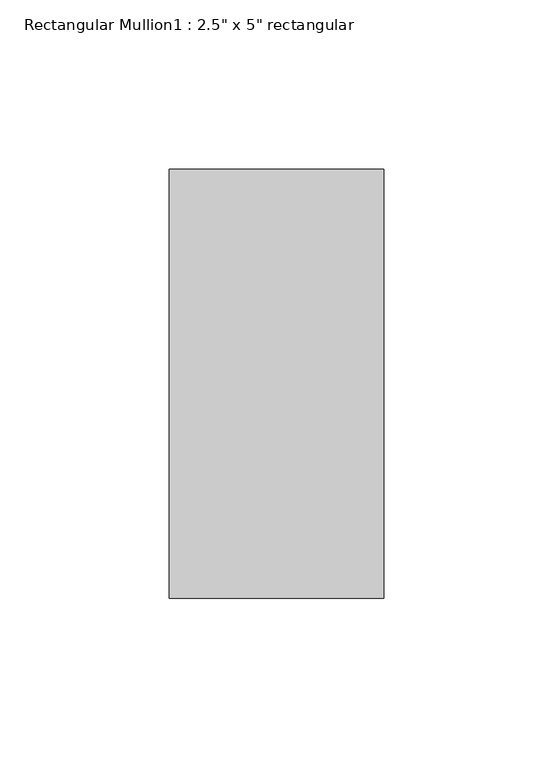
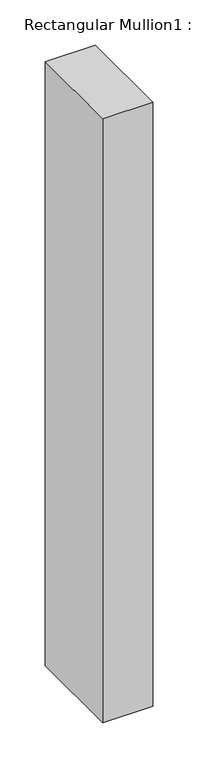
"""IFC4 building model written with IfcOpenShell, lengths in millimetres: member geometry."""

import ifcopenshell
import ifcopenshell.guid

model = None  # the IFC model being written
_history = None  # IfcOwnerHistory: only IFC2X3 demands one
_inside = {}  # id of a spatial element -> (the spatial element, [elements in it])
_under = {}  # id of a project, library or spatial element -> (it, [spatial elements below it])
_declared = {}  # id of a project -> (the project, [libraries it declares])
_typed = {}  # id of a type object -> (the type object, [elements of that type])
_made_of = {}  # id of a material, layer set ... -> (it, [elements and type objects made of it])


def new_model(schema):
    """Start an empty IFC model of exactly this schema.

    Asked for "IFC4X3", IfcOpenShell would pick the latest addendum, in which some entities
    have other attributes; the version numbers below select the first issue.
    IFC2X3 requires an IfcOwnerHistory on every rooted entity: one is made here for all.
    """
    global model, _history
    if schema == "IFC4X3":
        model = ifcopenshell.file(schema_version=(4, 3, 0, 0))
    else:
        model = ifcopenshell.file(schema=schema)
    _inside.clear()
    _under.clear()
    _declared.clear()
    _typed.clear()
    _made_of.clear()
    _history = None
    if model.schema == "IFC2X3":
        org = make("IfcOrganization", Name="unknown")
        user = make(
            "IfcPersonAndOrganization",
            ThePerson=make("IfcPerson", FamilyName="unknown"),
            TheOrganization=org,
        )
        app = make(
            "IfcApplication",
            ApplicationDeveloper=org,
            Version="unknown",
            ApplicationFullName="unknown",
            ApplicationIdentifier="unknown",
        )
        _history = make(
            "IfcOwnerHistory",
            OwningUser=user,
            OwningApplication=app,
            ChangeAction="ADDED",
            CreationDate=0,
        )
    return model


def make(cls, **values):
    """One entity of the class cls with the attributes given. An attribute that is None is left unset."""
    return model.create_entity(
        cls, **{name: value for name, value in values.items() if value is not None}
    )


def rooted(cls, **values):
    """An entity with a GlobalId (a new one), such as an element, a storey or a relation."""
    return make(cls, GlobalId=ifcopenshell.guid.new(), OwnerHistory=_history, **values)


def si_unit(unit_type, name, prefix=None):
    """IfcSIUnit, for example si_unit("LENGTHUNIT", "METRE", prefix="MILLI")."""
    return make("IfcSIUnit", UnitType=unit_type, Prefix=prefix, Name=name)


def assignment(units):
    """IfcUnitAssignment: the units of a project."""
    return None if units is None else make("IfcUnitAssignment", Units=units)


def point(xyz):
    """IfcCartesianPoint."""
    return None if xyz is None else make("IfcCartesianPoint", Coordinates=xyz)


def direction(xyz):
    """IfcDirection."""
    return None if xyz is None else make("IfcDirection", DirectionRatios=xyz)


def frame(location, z_axis=None, x_axis=None):
    """IfcAxis2Placement3D, a coordinate frame: its origin and axes. An axis left out is left unset."""
    return make(
        "IfcAxis2Placement3D",
        Location=point(location),
        Axis=direction(z_axis),
        RefDirection=direction(x_axis),
    )


def origin():
    """The frame at (0, 0, 0) with its axes left unset."""
    return frame((0.0, 0.0, 0.0))


def place(relative_to, where):
    """IfcLocalPlacement: puts the frame where relative to a parent placement (None: the world)."""
    return make(
        "IfcLocalPlacement", PlacementRelTo=relative_to, RelativePlacement=where
    )


def context(
    kind, dimensions, precision=None, world=None, true_north=None, identifier=None
):
    """IfcGeometricRepresentationContext, for example the 3D "Model" context."""
    return make(
        "IfcGeometricRepresentationContext",
        ContextIdentifier=identifier,
        ContextType=kind,
        CoordinateSpaceDimension=dimensions,
        Precision=precision,
        WorldCoordinateSystem=world,
        TrueNorth=true_north,
    )


def project(units=None, contexts=None):
    """IfcProject with its units and contexts."""
    return rooted(
        "IfcProject",
        Name="project",
        RepresentationContexts=contexts,
        UnitsInContext=assignment(units),
    )


def spatial(cls, under=None, at=None, **own):
    """A site, building, storey or space (cls), placed at a placement, below another one or the project."""
    s = rooted(cls, ObjectPlacement=at, **own)
    if under is not None:
        _under.setdefault(under.id(), (under, []))[1].append(s)
    return s


def polyline(points):
    """IfcPolyline through the points."""
    return make("IfcPolyline", Points=[point(p) for p in points])


def outline(outer, holes=None, kind="AREA"):
    """IfcArbitraryClosedProfileDef: a profile drawn as a closed curve; with holes, ...WithVoids."""
    if holes is None:
        return make("IfcArbitraryClosedProfileDef", ProfileType=kind, OuterCurve=outer)
    return make(
        "IfcArbitraryProfileDefWithVoids",
        ProfileType=kind,
        OuterCurve=outer,
        InnerCurves=holes,
    )


def extrude(swept, where, along, depth):
    """IfcExtrudedAreaSolid: the profile swept, set in the frame where, extruded along a direction by depth."""
    return make(
        "IfcExtrudedAreaSolid",
        SweptArea=swept,
        Position=where,
        ExtrudedDirection=direction(along),
        Depth=depth,
    )


def shape(context_of_items, identifier, shape_type, items):
    """IfcShapeRepresentation: the items that make up one representation, for example the "Body"."""
    return make(
        "IfcShapeRepresentation",
        ContextOfItems=context_of_items,
        RepresentationIdentifier=identifier,
        RepresentationType=shape_type,
        Items=items,
    )


def source(mapping_origin, context_of_items, identifier, shape_type, items):
    """IfcRepresentationMap: a shape defined once, which mapped items show again and again."""
    return make(
        "IfcRepresentationMap",
        MappingOrigin=mapping_origin,
        MappedRepresentation=shape(context_of_items, identifier, shape_type, items),
    )


def transform(
    local_origin,
    x_axis=None,
    y_axis=None,
    z_axis=None,
    scale=None,
    scale2=None,
    scale3=None,
    uniform=True,
):
    """IfcCartesianTransformationOperator3D, or its non-uniform kind. x_axis, y_axis, z_axis: its Axis1, 2, 3."""
    if uniform:
        return make(
            "IfcCartesianTransformationOperator3D",
            Axis1=direction(x_axis),
            Axis2=direction(y_axis),
            LocalOrigin=point(local_origin),
            Scale=scale,
            Axis3=direction(z_axis),
        )
    return make(
        "IfcCartesianTransformationOperator3DnonUniform",
        Axis1=direction(x_axis),
        Axis2=direction(y_axis),
        LocalOrigin=point(local_origin),
        Scale=scale,
        Axis3=direction(z_axis),
        Scale2=scale2,
        Scale3=scale3,
    )


def mapped(mapping_source, mapping_target):
    """IfcMappedItem: shows the shape of a source again, moved by a transform."""
    return make(
        "IfcMappedItem", MappingSource=mapping_source, MappingTarget=mapping_target
    )


def made_of(thing, what):
    """Note that an element or type object is made of a material, layer set ...; save() writes the relation."""
    if what is not None:
        _made_of.setdefault(what.id(), (what, []))[1].append(thing)
    return thing


def element(
    cls,
    number,
    at=None,
    inside=None,
    cuts=None,
    type_object=None,
    material=None,
    context=None,
    identifier="Body",
    shape_type=None,
    held_by="IfcProductDefinitionShape",
    body=None,
    shapes=None,
    **own,
):
    """One element of the class cls, such as IfcWall. Its Tag is "e" and its number.

    at: its placement. inside: the storey or other place that contains it. cuts: it is an
    opening in that element (IfcRelVoidsElement). A single representation is given by context,
    identifier, shape_type and body (its items); several are given by shapes. held_by: the class
    of the entity that holds the representations. save() writes the other relations.
    """
    e = rooted(cls, Tag="e%d" % number, ObjectPlacement=at, **own)
    if body is not None:
        shapes = [shape(context, identifier, shape_type, body)]
    if shapes is not None:
        e.Representation = make(held_by, Representations=shapes)
    if inside is not None:
        _inside.setdefault(inside.id(), (inside, []))[1].append(e)
    if cuts is not None:
        rooted(
            "IfcRelVoidsElement", RelatingBuildingElement=cuts, RelatedOpeningElement=e
        )
    if type_object is not None:
        _typed.setdefault(type_object.id(), (type_object, []))[1].append(e)
    return made_of(e, material)


def aggregate(whole, parts):
    """IfcRelAggregates: a whole, such as a stair, and the parts it consists of."""
    return rooted("IfcRelAggregates", RelatingObject=whole, RelatedObjects=parts)


def save(model, path):
    """Write the relations noted so far, then the file.

    IfcRelAggregates (storeys below a building ...), IfcRelContainedInSpatialStructure (elements
    in a storey), IfcRelDefinesByType, IfcRelAssociatesMaterial and IfcRelDeclares: one each for
    every whole, place, type object, material and project.
    """
    for whole, parts in _under.values():
        aggregate(whole, parts)
    for where, things in _inside.values():
        rooted(
            "IfcRelContainedInSpatialStructure",
            RelatedElements=things,
            RelatingStructure=where,
        )
    for kind, things in _typed.values():
        rooted("IfcRelDefinesByType", RelatedObjects=things, RelatingType=kind)
    for what, things in _made_of.values():
        rooted("IfcRelAssociatesMaterial", RelatedObjects=things, RelatingMaterial=what)
    for by, libraries in _declared.values():
        rooted("IfcRelDeclares", RelatingContext=by, RelatedDefinitions=libraries)
    model.write(path)


def member_7227ddca(model_context):
    return source(origin(), model_context, "Body", "SweptSolid", [
        extrude(outline(polyline([(0.0, 63.5), (0.0, -63.5), (-63.5, -63.5), (-63.5, 63.5), (0.0, 63.5)])), frame((0.0, 0.0, -813.7989637), z_axis=(0.0, 0.0, 1.0), x_axis=(1.0, 0.0, 0.0)), (0.0, 0.0, 1.0), 813.7989637),
    ])


if __name__ == "__main__":
    model = new_model("IFC4")
    model_context = context("Model", 3, world=origin())
    ifc_project = project(units=[si_unit("LENGTHUNIT", "METRE", prefix="MILLI")], contexts=[model_context])
    site = spatial("IfcSite", under=ifc_project)
    building = spatial("IfcBuilding", under=site)
    placement = place(None, origin())
    member_shape = member_7227ddca(model_context)
    element("IfcMember", 1, ObjectType="Rectangular Mullion1 : 2.5\" x 5\" rectangular", at=placement, inside=building, context=model_context, shape_type="MappedRepresentation", body=[
        mapped(member_shape, transform((0.0, 0.0, 0.0), x_axis=(1.0, 0.0, 0.0), y_axis=(0.0, 1.0, 0.0), z_axis=(0.0, 0.0, 1.0))),
    ])
    save(model, "model.ifc")

# Revit data of these elements
# Type "Rectangular Mullion1 : 2.5\" x 5\" rectangular"
#   built-in parameter 1007304 = 0.416667 (stored number, unit not read)
#   built-in parameter 1007301 = 0.104167 (stored number, unit not read)
#   built-in parameter 1007300 = 0.104167 (stored number, unit not read)
# Element 1 (IfcMember, "Rectangular Mullion1 : 2.5\" x 5\" rectangular")
#   Materials on its faces: "support-frame"
# Materials
#   "support-frame": class "Unassigned", colour RGB 233 233 233, transparency 0, Cost = 0
